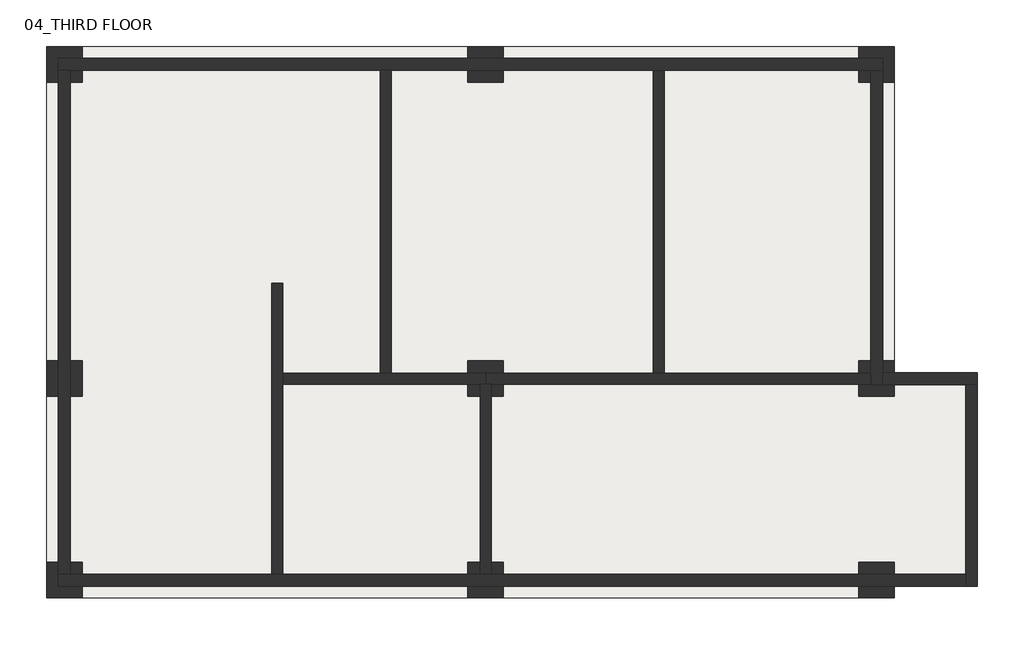
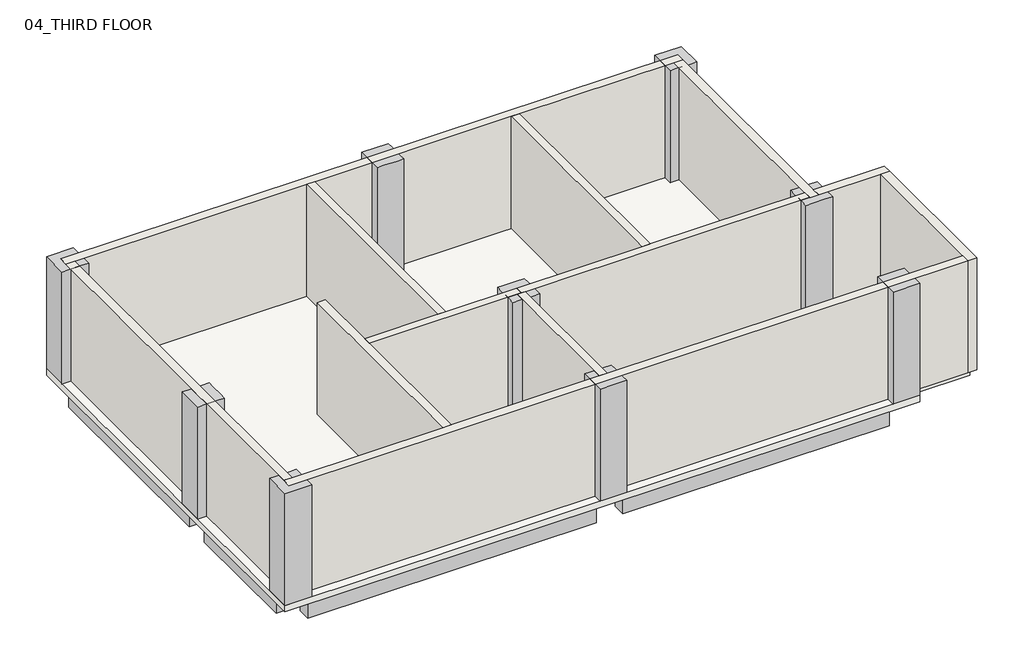
# One storey: 12 beams, 12 walls, 9 columns, 1 slab.
"""IFC4 building model written with IfcOpenShell, lengths in millimetres."""

from ifc_helpers import new_model, si_unit, frame, origin, place, context, project, spatial, polyline, outline, extrude, faceted_brep, element, save

model = new_model("IFC4")

# Units and contexts
model_context = context("Model", 3, world=origin())
ifc_project = project(units=[si_unit("LENGTHUNIT", "METRE", prefix="MILLI")], contexts=[model_context])

# Site, building, storey
site = spatial("IfcSite", under=ifc_project)
building = spatial("IfcBuilding", under=site)
storey = spatial("IfcBuildingStorey", under=building, Name="04_THIRD FLOOR", Elevation=8639.9618634)

# Beams
placement = place(None, origin())
element("IfcBeam", 1, ObjectType="RC Beam_Rectangular : H_SB_AR_S16_B300xH600", at=placement, inside=storey, context=model_context, shape_type="SweptSolid", body=[
    extrude(outline(polyline([(300.0, 1049.5208589), (300.0, 1349.5208589), (6800.0, 1349.5208589), (6800.0, 1049.5208589), (300.0, 1049.5208589)])), frame((0.0, 0.0, 8039.9618634), z_axis=(0.0, 0.0, 1.0), x_axis=(1.0, 0.0, 0.0)), (0.0, 0.0, 1.0), 450.0),
])
element("IfcBeam", 2, ObjectType="RC Beam_Rectangular : H_SB_AR_S16_B300xH600", at=placement, inside=storey, context=model_context, shape_type="SweptSolid", body=[
    extrude(outline(polyline([(7400.0, 1049.5208589), (7400.0, 1349.5208589), (13400.0, 1349.5208589), (13400.0, 1049.5208589), (7400.0, 1049.5208589)])), frame((0.0, 0.0, 8039.9618634), z_axis=(0.0, 0.0, 1.0), x_axis=(1.0, 0.0, 0.0)), (0.0, 0.0, 1.0), 450.0),
])
element("IfcBeam", 3, ObjectType="RC Beam_Rectangular : H_SB_AR_S16_B300xH600", at=placement, inside=storey, context=model_context, shape_type="SweptSolid", body=[
    extrude(outline(polyline([(300.0, 6349.5208589), (300.0, 6649.5208589), (6800.0, 6649.5208589), (6800.0, 6349.5208589), (300.0, 6349.5208589)])), frame((0.0, 0.0, 8039.9618634), z_axis=(0.0, 0.0, 1.0), x_axis=(1.0, 0.0, 0.0)), (0.0, 0.0, 1.0), 450.0),
])
element("IfcBeam", 4, ObjectType="RC Beam_Rectangular : H_SB_AR_S16_B300xH600", at=placement, inside=storey, context=model_context, shape_type="SweptSolid", body=[
    extrude(outline(polyline([(7400.0, 6349.5208589), (7400.0, 6649.5208589), (13400.0, 6649.5208589), (13400.0, 6349.5208589), (7400.0, 6349.5208589)])), frame((0.0, 0.0, 8039.9618634), z_axis=(0.0, 0.0, 1.0), x_axis=(1.0, 0.0, 0.0)), (0.0, 0.0, 1.0), 450.0),
])
element("IfcBeam", 5, ObjectType="RC Beam_Rectangular : H_SB_AR_S16_B300xH600", at=placement, inside=storey, context=model_context, shape_type="SweptSolid", body=[
    extrude(outline(polyline([(300.0, -2350.4791411), (300.0, -2050.4791411), (6800.0, -2050.4791411), (6800.0, -2350.4791411), (300.0, -2350.4791411)])), frame((0.0, 0.0, 8039.9618634), z_axis=(0.0, 0.0, 1.0), x_axis=(1.0, 0.0, 0.0)), (0.0, 0.0, 1.0), 450.0),
])
element("IfcBeam", 6, ObjectType="RC Beam_Rectangular : H_SB_AR_S16_B300xH600", at=placement, inside=storey, context=model_context, shape_type="SweptSolid", body=[
    extrude(outline(polyline([(7400.0, -2350.4791411), (7400.0, -2050.4791411), (13400.0, -2050.4791411), (13400.0, -2350.4791411), (7400.0, -2350.4791411)])), frame((0.0, 0.0, 8039.9618634), z_axis=(0.0, 0.0, 1.0), x_axis=(1.0, 0.0, 0.0)), (0.0, 0.0, 1.0), 450.0),
])
element("IfcBeam", 7, ObjectType="RC Beam_Rectangular : H_SB_AR_S16_B300xH600", at=placement, inside=storey, context=model_context, shape_type="SweptSolid", body=[
    extrude(outline(polyline([(-150.0, 899.5208589), (150.0, 899.5208589), (150.0, -1900.4791411), (-150.0, -1900.4791411), (-150.0, 899.5208589)])), frame((0.0, 0.0, 8039.9618634), z_axis=(0.0, 0.0, 1.0), x_axis=(1.0, 0.0, 0.0)), (0.0, 0.0, 1.0), 450.0),
])
element("IfcBeam", 8, ObjectType="RC Beam_Rectangular : H_SB_AR_S16_B300xH600", at=placement, inside=storey, context=model_context, shape_type="SweptSolid", body=[
    extrude(outline(polyline([(150.0, 1499.5208589), (-150.0, 1499.5208589), (-150.0, 6199.5208589), (150.0, 6199.5208589), (150.0, 1499.5208589)])), frame((0.0, 0.0, 8039.9618634), z_axis=(0.0, 0.0, 1.0), x_axis=(1.0, 0.0, 0.0)), (0.0, 0.0, 1.0), 450.0),
])
element("IfcBeam", 9, ObjectType="RC Beam_Rectangular : H_SB_AR_S16_B300xH600", at=placement, inside=storey, context=model_context, shape_type="SweptSolid", body=[
    extrude(outline(polyline([(6950.0, 899.5208589), (7250.0, 899.5208589), (7250.0, -1900.4791411), (6950.0, -1900.4791411), (6950.0, 899.5208589)])), frame((0.0, 0.0, 8039.9618634), z_axis=(0.0, 0.0, 1.0), x_axis=(1.0, 0.0, 0.0)), (0.0, 0.0, 1.0), 450.0),
])
element("IfcBeam", 10, ObjectType="RC Beam_Rectangular : H_SB_AR_S16_B300xH600", at=placement, inside=storey, context=model_context, shape_type="SweptSolid", body=[
    extrude(outline(polyline([(7250.0, 1499.5208589), (6950.0, 1499.5208589), (6950.0, 6199.5208589), (7250.0, 6199.5208589), (7250.0, 1499.5208589)])), frame((0.0, 0.0, 8039.9618634), z_axis=(0.0, 0.0, 1.0), x_axis=(1.0, 0.0, 0.0)), (0.0, 0.0, 1.0), 450.0),
])
element("IfcBeam", 11, ObjectType="RC Beam_Rectangular : H_SB_AR_S16_B300xH600", at=placement, inside=storey, context=model_context, shape_type="SweptSolid", body=[
    extrude(outline(polyline([(13550.0, 899.5208589), (13850.0, 899.5208589), (13850.0, -1900.4791411), (13550.0, -1900.4791411), (13550.0, 899.5208589)])), frame((0.0, 0.0, 8039.9618634), z_axis=(0.0, 0.0, 1.0), x_axis=(1.0, 0.0, 0.0)), (0.0, 0.0, 1.0), 450.0),
])
element("IfcBeam", 12, ObjectType="RC Beam_Rectangular : H_SB_AR_S16_B300xH600", at=placement, inside=storey, context=model_context, shape_type="SweptSolid", body=[
    extrude(outline(polyline([(13850.0, 1499.5208589), (13550.0, 1499.5208589), (13550.0, 6199.5208589), (13850.0, 6199.5208589), (13850.0, 1499.5208589)])), frame((0.0, 0.0, 8039.9618634), z_axis=(0.0, 0.0, 1.0), x_axis=(1.0, 0.0, 0.0)), (0.0, 0.0, 1.0), 450.0),
])

# Columns
element("IfcColumn", 13, ObjectType="RC_Column_Rectangular : H_SC_AR_S15_W600xL600", at=placement, inside=storey, context=model_context, shape_type="Brep", body=[
    faceted_brep([(300.0, 1499.5208589, 8639.9618634), (300.0, 899.5208589, 8639.9618634), (-300.0, 899.5208589, 8639.9618634), (-300.0, 1499.5208589, 8639.9618634), (300.0, 1499.5208589, 11309.9618634), (300.0, 1349.5208589, 11309.9618634), (300.0, 1049.5208589, 11309.9618634), (300.0, 899.5208589, 11309.9618634), (150.0, 899.5208589, 11309.9618634), (-150.0, 899.5208589, 11309.9618634), (-300.0, 899.5208589, 11309.9618634), (-300.0, 1499.5208589, 11309.9618634), (-150.0, 1499.5208589, 11309.9618634), (150.0, 1499.5208589, 11309.9618634)], [[[0, 1, 2, 3]], [[4, 5, 6, 7, 1, 0]], [[7, 8, 9, 10, 2, 1]], [[10, 11, 3, 2]], [[11, 12, 13, 4, 0, 3]], [[4, 13, 12, 11, 10, 9, 8, 7, 6, 5]]]),
])
element("IfcColumn", 14, ObjectType="RC_Column_Rectangular : H_SC_AR_S15_W600xL600", at=placement, inside=storey, context=model_context, shape_type="Brep", body=[
    faceted_brep([(7400.0, 1499.5208589, 8639.9618634), (7400.0, 899.5208589, 8639.9618634), (6800.0, 899.5208589, 8639.9618634), (6800.0, 1499.5208589, 8639.9618634), (7400.0, 1499.5208589, 11309.9618634), (7400.0, 1349.5208589, 11309.9618634), (7400.0, 1049.5208589, 11309.9618634), (7400.0, 899.5208589, 11309.9618634), (7250.0, 899.5208589, 11309.9618634), (6950.0, 899.5208589, 11309.9618634), (6800.0, 899.5208589, 11309.9618634), (6800.0, 1049.5208589, 11309.9618634), (6800.0, 1349.5208589, 11309.9618634), (6800.0, 1499.5208589, 11309.9618634), (6950.0, 1499.5208589, 11309.9618634), (7250.0, 1499.5208589, 11309.9618634)], [[[0, 1, 2, 3]], [[4, 5, 6, 7, 1, 0]], [[7, 8, 9, 10, 2, 1]], [[10, 11, 12, 13, 3, 2]], [[13, 14, 15, 4, 0, 3]], [[4, 15, 14, 13, 12, 11, 10, 9, 8, 7, 6, 5]]]),
])
element("IfcColumn", 15, ObjectType="RC_Column_Rectangular : H_SC_AR_S15_W600xL600", at=placement, inside=storey, context=model_context, shape_type="Brep", body=[
    faceted_brep([(14000.0, 1499.5208589, 8639.9618634), (14000.0, 899.5208589, 8639.9618634), (13400.0, 899.5208589, 8639.9618634), (13400.0, 1499.5208589, 8639.9618634), (14000.0, 1499.5208589, 11309.9618634), (14000.0, 1199.5208589, 11309.9618634), (14000.0, 899.5208589, 11309.9618634), (13850.0, 899.5208589, 11309.9618634), (13550.0, 899.5208589, 11309.9618634), (13400.0, 899.5208589, 11309.9618634), (13400.0, 1049.5208589, 11309.9618634), (13400.0, 1349.5208589, 11309.9618634), (13400.0, 1499.5208589, 11309.9618634), (13550.0, 1499.5208589, 11309.9618634), (13850.0, 1499.5208589, 11309.9618634)], [[[0, 1, 2, 3]], [[4, 5, 6, 1, 0]], [[6, 7, 8, 9, 2, 1]], [[9, 10, 11, 12, 3, 2]], [[12, 13, 14, 4, 0, 3]], [[4, 14, 13, 12, 11, 10, 9, 8, 7, 6, 5]]]),
])
element("IfcColumn", 16, ObjectType="RC_Column_Rectangular : H_SC_AR_S15_W600xL600", at=placement, inside=storey, context=model_context, shape_type="Brep", body=[
    faceted_brep([(300.0, 6799.5208589, 8639.9618634), (300.0, 6199.5208589, 8639.9618634), (-300.0, 6199.5208589, 8639.9618634), (-300.0, 6799.5208589, 8639.9618634), (300.0, 6799.5208589, 11309.9618634), (300.0, 6649.5208589, 11309.9618634), (300.0, 6349.5208589, 11309.9618634), (300.0, 6199.5208589, 11309.9618634), (150.0, 6199.5208589, 11309.9618634), (-150.0, 6199.5208589, 11309.9618634), (-300.0, 6199.5208589, 11309.9618634), (-300.0, 6799.5208589, 11309.9618634)], [[[0, 1, 2, 3]], [[4, 5, 6, 7, 1, 0]], [[7, 8, 9, 10, 2, 1]], [[10, 11, 3, 2]], [[11, 4, 0, 3]], [[4, 11, 10, 9, 8, 7, 6, 5]]]),
])
element("IfcColumn", 17, ObjectType="RC_Column_Rectangular : H_SC_AR_S15_W600xL600", at=placement, inside=storey, context=model_context, shape_type="Brep", body=[
    faceted_brep([(7400.0, 6799.5208589, 8639.9618634), (7400.0, 6199.5208589, 8639.9618634), (6800.0, 6199.5208589, 8639.9618634), (6800.0, 6799.5208589, 8639.9618634), (7400.0, 6799.5208589, 11309.9618634), (7400.0, 6649.5208589, 11309.9618634), (7400.0, 6349.5208589, 11309.9618634), (7400.0, 6199.5208589, 11309.9618634), (7250.0, 6199.5208589, 11309.9618634), (6950.0, 6199.5208589, 11309.9618634), (6800.0, 6199.5208589, 11309.9618634), (6800.0, 6349.5208589, 11309.9618634), (6800.0, 6649.5208589, 11309.9618634), (6800.0, 6799.5208589, 11309.9618634)], [[[0, 1, 2, 3]], [[4, 5, 6, 7, 1, 0]], [[7, 8, 9, 10, 2, 1]], [[10, 11, 12, 13, 3, 2]], [[13, 4, 0, 3]], [[4, 13, 12, 11, 10, 9, 8, 7, 6, 5]]]),
])
element("IfcColumn", 18, ObjectType="RC_Column_Rectangular : H_SC_AR_S15_W600xL600", at=placement, inside=storey, context=model_context, shape_type="Brep", body=[
    faceted_brep([(14000.0, 6799.5208589, 8639.9618634), (14000.0, 6199.5208589, 8639.9618634), (13400.0, 6199.5208589, 8639.9618634), (13400.0, 6799.5208589, 8639.9618634), (14000.0, 6799.5208589, 11309.9618634), (14000.0, 6199.5208589, 11309.9618634), (13850.0, 6199.5208589, 11309.9618634), (13550.0, 6199.5208589, 11309.9618634), (13400.0, 6199.5208589, 11309.9618634), (13400.0, 6349.5208589, 11309.9618634), (13400.0, 6649.5208589, 11309.9618634), (13400.0, 6799.5208589, 11309.9618634)], [[[0, 1, 2, 3]], [[4, 5, 1, 0]], [[5, 6, 7, 8, 2, 1]], [[8, 9, 10, 11, 3, 2]], [[11, 4, 0, 3]], [[4, 11, 10, 9, 8, 7, 6, 5]]]),
])
element("IfcColumn", 19, ObjectType="RC_Column_Rectangular : H_SC_AR_S15_W600xL600", at=placement, inside=storey, context=model_context, shape_type="Brep", body=[
    faceted_brep([(300.0, -1900.4791411, 8639.9618634), (300.0, -2500.4791411, 8639.9618634), (-300.0, -2500.4791411, 8639.9618634), (-300.0, -1900.4791411, 8639.9618634), (300.0, -1900.4791411, 11309.9618634), (300.0, -2050.4791411, 11309.9618634), (300.0, -2350.4791411, 11309.9618634), (300.0, -2500.4791411, 11309.9618634), (-300.0, -2500.4791411, 11309.9618634), (-300.0, -1900.4791411, 11309.9618634), (-150.0, -1900.4791411, 11309.9618634), (150.0, -1900.4791411, 11309.9618634)], [[[0, 1, 2, 3]], [[4, 5, 6, 7, 1, 0]], [[7, 8, 2, 1]], [[8, 9, 3, 2]], [[9, 10, 11, 4, 0, 3]], [[4, 11, 10, 9, 8, 7, 6, 5]]]),
])
element("IfcColumn", 20, ObjectType="RC_Column_Rectangular : H_SC_AR_S15_W600xL600", at=placement, inside=storey, context=model_context, shape_type="Brep", body=[
    faceted_brep([(7400.0, -1900.4791411, 8639.9618634), (7400.0, -2500.4791411, 8639.9618634), (6800.0, -2500.4791411, 8639.9618634), (6800.0, -1900.4791411, 8639.9618634), (7400.0, -1900.4791411, 11309.9618634), (7400.0, -2050.4791411, 11309.9618634), (7400.0, -2350.4791411, 11309.9618634), (7400.0, -2500.4791411, 11309.9618634), (7100.0, -2500.4791411, 11309.9618634), (6800.0, -2500.4791411, 11309.9618634), (6800.0, -2350.4791411, 11309.9618634), (6800.0, -2050.4791411, 11309.9618634), (6800.0, -1900.4791411, 11309.9618634), (6950.0, -1900.4791411, 11309.9618634), (7250.0, -1900.4791411, 11309.9618634)], [[[0, 1, 2, 3]], [[4, 5, 6, 7, 1, 0]], [[7, 8, 9, 2, 1]], [[9, 10, 11, 12, 3, 2]], [[12, 13, 14, 4, 0, 3]], [[4, 14, 13, 12, 11, 10, 9, 8, 7, 6, 5]]]),
])
element("IfcColumn", 21, ObjectType="RC_Column_Rectangular : H_SC_AR_S15_W600xL600", at=placement, inside=storey, context=model_context, shape_type="Brep", body=[
    faceted_brep([(14000.0, -1900.4791411, 8639.9618634), (14000.0, -2500.4791411, 8639.9618634), (13400.0, -2500.4791411, 8639.9618634), (13400.0, -1900.4791411, 8639.9618634), (14000.0, -1900.4791411, 11309.9618634), (14000.0, -2500.4791411, 11309.9618634), (13400.0, -2500.4791411, 11309.9618634), (13400.0, -2350.4791411, 11309.9618634), (13400.0, -2050.4791411, 11309.9618634), (13400.0, -1900.4791411, 11309.9618634), (13550.0, -1900.4791411, 11309.9618634), (13850.0, -1900.4791411, 11309.9618634)], [[[0, 1, 2, 3]], [[4, 5, 1, 0]], [[5, 6, 2, 1]], [[6, 7, 8, 9, 3, 2]], [[9, 10, 11, 4, 0, 3]], [[4, 11, 10, 9, 8, 7, 6, 5]]]),
])

# Slab
element("IfcSlab", 22, ObjectType="H_FL_AR_S17_RC Slab T150", at=placement, inside=storey, context=model_context, shape_type="SweptSolid", body=[
    extrude(outline(polyline([(14000.0, 1199.5208589), (15300.0, 1199.5208589), (15300.0, -2200.4791411), (14000.0, -2200.4791411), (14000.0, -2500.4791411), (-300.0, -2500.4791411), (-300.0, 6799.5208589), (14000.0, 6799.5208589), (14000.0, 1199.5208589)])), frame((0.0, 0.0, 8489.9618634), z_axis=(0.0, 0.0, 1.0), x_axis=(1.0, 0.0, 0.0)), (0.0, 0.0, 1.0), 150.0),
])

# Walls
element("IfcWall", 23, ObjectType="H_WA_AR_B02_Ext Wall_RC T200", at=placement, inside=storey, context=model_context, shape_type="Brep", body=[
    faceted_brep([(-100.0, 6399.5208589, 8639.9618634), (100.0, 6399.5208589, 8639.9618634), (5325.5, 6399.5208589, 8639.9618634), (5509.5, 6399.5208589, 8639.9618634), (9935.0, 6399.5208589, 8639.9618634), (10119.0, 6399.5208589, 8639.9618634), (13600.0, 6399.5208589, 8639.9618634), (13800.0, 6399.5208589, 8639.9618634), (13800.0, 6399.5208589, 11309.9618634), (13600.0, 6399.5208589, 11309.9618634), (10119.0, 6399.5208589, 11309.9618634), (9935.0, 6399.5208589, 11309.9618634), (5509.5, 6399.5208589, 11309.9618634), (5325.5, 6399.5208589, 11309.9618634), (100.0, 6399.5208589, 11309.9618634), (-100.0, 6399.5208589, 11309.9618634), (-100.0, 6599.5208589, 8639.9618634), (-100.0, 6599.5208589, 11309.9618634), (13800.0, 6599.5208589, 11309.9618634), (13800.0, 6599.5208589, 8639.9618634)], [[[0, 1, 2, 3, 4, 5, 6, 7, 8, 9, 10, 11, 12, 13, 14, 15]], [[16, 17, 18, 19]], [[7, 6, 5, 4, 3, 2, 1, 0, 16, 19]], [[15, 14, 13, 12, 11, 10, 9, 8, 18, 17]], [[8, 7, 19, 18]], [[0, 15, 17, 16]]]),
])
element("IfcWall", 24, ObjectType="H_WA_AR_B02_Ext Wall_RC T200", at=placement, inside=storey, context=model_context, shape_type="Brep", body=[
    faceted_brep([(13600.0, 6399.5208589, 8639.9618634), (13600.0, 1286.5208589, 8639.9618634), (13600.0, 1102.5208589, 8639.9618634), (13600.0, 1099.5208589, 8639.9618634), (13600.0, 1099.5208589, 11309.9618634), (13600.0, 1102.5208589, 11309.9618634), (13600.0, 1286.5208589, 11309.9618634), (13600.0, 6399.5208589, 11309.9618634), (13800.0, 6399.5208589, 8639.9618634), (13800.0, 6399.5208589, 11309.9618634), (13800.0, 1299.5208589, 11309.9618634), (13800.0, 1099.5208589, 11309.9618634), (13800.0, 1099.5208589, 8639.9618634), (13800.0, 1299.5208589, 8639.9618634)], [[[0, 1, 2, 3, 4, 5, 6, 7]], [[8, 9, 10, 11, 12, 13]], [[3, 2, 1, 0, 8, 13, 12]], [[7, 6, 5, 4, 11, 10, 9]], [[0, 7, 9, 8]], [[4, 3, 12, 11]]]),
])
element("IfcWall", 25, ObjectType="H_WA_AR_B02_Ext Wall_RC T200", at=placement, inside=storey, context=model_context, shape_type="Brep", body=[
    faceted_brep([(13800.0, 1099.5208589, 8639.9618634), (15200.0, 1099.5208589, 8639.9618634), (15400.0, 1099.5208589, 8639.9618634), (15400.0, 1099.5208589, 11309.9618634), (15200.0, 1099.5208589, 11309.9618634), (13800.0, 1099.5208589, 11309.9618634), (13800.0, 1299.5208589, 8639.9618634), (13800.0, 1299.5208589, 11309.9618634), (15400.0, 1299.5208589, 11309.9618634), (15400.0, 1299.5208589, 8639.9618634)], [[[0, 1, 2, 3, 4, 5]], [[6, 7, 8, 9]], [[2, 1, 0, 6, 9]], [[5, 4, 3, 8, 7]], [[0, 5, 7, 6]], [[3, 2, 9, 8]]]),
])
element("IfcWall", 26, ObjectType="H_WA_AR_B02_Ext Wall_RC T200", at=placement, inside=storey, context=model_context, shape_type="Brep", body=[
    faceted_brep([(15200.0, 1099.5208589, 8639.9618634), (15200.0, -2100.4791411, 8639.9618634), (15200.0, -2300.4791411, 8639.9618634), (15200.0, -2300.4791411, 11309.9618634), (15200.0, -2100.4791411, 11309.9618634), (15200.0, 1099.5208589, 11309.9618634), (15400.0, 1099.5208589, 8639.9618634), (15400.0, 1099.5208589, 11309.9618634), (15400.0, -2300.4791411, 11309.9618634), (15400.0, -2300.4791411, 8639.9618634)], [[[0, 1, 2, 3, 4, 5]], [[6, 7, 8, 9]], [[2, 1, 0, 6, 9]], [[5, 4, 3, 8, 7]], [[0, 5, 7, 6]], [[3, 2, 9, 8]]]),
])
element("IfcWall", 27, ObjectType="H_WA_AR_B02_Ext Wall_RC T200", at=placement, inside=storey, context=model_context, shape_type="Brep", body=[
    faceted_brep([(15200.0, -2100.4791411, 8639.9618634), (7197.0, -2100.4791411, 8639.9618634), (7013.0, -2100.4791411, 8639.9618634), (3680.0, -2100.4791411, 8639.9618634), (3496.0, -2100.4791411, 8639.9618634), (100.0, -2100.4791411, 8639.9618634), (-100.0, -2100.4791411, 8639.9618634), (-100.0, -2100.4791411, 11309.9618634), (100.0, -2100.4791411, 11309.9618634), (3496.0, -2100.4791411, 11309.9618634), (3680.0, -2100.4791411, 11309.9618634), (7013.0, -2100.4791411, 11309.9618634), (7197.0, -2100.4791411, 11309.9618634), (15200.0, -2100.4791411, 11309.9618634), (15200.0, -2300.4791411, 8639.9618634), (15200.0, -2300.4791411, 11309.9618634), (-100.0, -2300.4791411, 11309.9618634), (-100.0, -2300.4791411, 8639.9618634)], [[[0, 1, 2, 3, 4, 5, 6, 7, 8, 9, 10, 11, 12, 13]], [[14, 15, 16, 17]], [[6, 5, 4, 3, 2, 1, 0, 14, 17]], [[13, 12, 11, 10, 9, 8, 7, 16, 15]], [[0, 13, 15, 14]], [[7, 6, 17, 16]]]),
])
element("IfcWall", 28, ObjectType="H_WA_AR_B02_Ext Wall_RC T200", at=placement, inside=storey, context=model_context, shape_type="SweptSolid", body=[
    extrude(outline(polyline([(100.0, 6399.5208589), (100.0, -2100.4791411), (-100.0, -2100.4791411), (-100.0, 6399.5208589), (100.0, 6399.5208589)])), frame((0.0, 0.0, 8639.9618634), z_axis=(0.0, 0.0, 1.0), x_axis=(1.0, 0.0, 0.0)), (0.0, 0.0, 1.0), 2670.0),
])
element("IfcWall", 29, ObjectType="H_WA_AR_B02_Int Wall_Block T150", at=placement, inside=storey, context=model_context, shape_type="Brep", body=[
    faceted_brep([(7197.0, -2100.4791411, 8639.9618634), (7197.0, 1102.5208589, 8639.9618634), (7197.0, 1102.5208589, 11309.9618634), (7197.0, -2100.4791411, 11309.9618634), (7013.0, -2100.4791411, 8639.9618634), (7013.0, -2100.4791411, 11309.9618634), (7013.0, 1102.5208589, 11309.9618634), (7013.0, 1102.5208589, 8639.9618634), (7105.0, 1102.5208589, 8639.9618634), (7105.0, 1102.5208589, 11309.9618634)], [[[0, 1, 2, 3]], [[4, 5, 6, 7]], [[1, 0, 4, 7, 8]], [[3, 2, 9, 6, 5]], [[0, 3, 5, 4]], [[2, 1, 8, 7, 6, 9]]]),
])
element("IfcWall", 30, ObjectType="H_WA_AR_B02_Int Wall_Block T150", at=placement, inside=storey, context=model_context, shape_type="Brep", body=[
    faceted_brep([(7105.0, 1102.5208589, 8639.9618634), (7197.0, 1102.5208589, 8639.9618634), (13600.0, 1102.5208589, 8639.9618634), (13600.0, 1102.5208589, 11309.9618634), (7197.0, 1102.5208589, 11309.9618634), (7105.0, 1102.5208589, 11309.9618634), (7105.0, 1286.5208589, 8639.9618634), (7105.0, 1286.5208589, 11309.9618634), (9935.0, 1286.5208589, 11309.9618634), (10119.0, 1286.5208589, 11309.9618634), (13600.0, 1286.5208589, 11309.9618634), (13600.0, 1286.5208589, 8639.9618634), (10119.0, 1286.5208589, 8639.9618634), (9935.0, 1286.5208589, 8639.9618634)], [[[0, 1, 2, 3, 4, 5]], [[6, 7, 8, 9, 10, 11, 12, 13]], [[2, 1, 0, 6, 13, 12, 11]], [[5, 4, 3, 10, 9, 8, 7]], [[0, 5, 7, 6]], [[3, 2, 11, 10]]]),
])
element("IfcWall", 31, ObjectType="H_WA_AR_B02_Int Wall_Block T150", at=placement, inside=storey, context=model_context, shape_type="Brep", body=[
    faceted_brep([(3496.0, 2811.5208589, 8639.9618634), (3496.0, -2100.4791411, 8639.9618634), (3496.0, -2100.4791411, 11309.9618634), (3496.0, 2811.5208589, 11309.9618634), (3680.0, 2811.5208589, 8639.9618634), (3680.0, 2811.5208589, 11309.9618634), (3680.0, 1286.5208589, 11309.9618634), (3680.0, 1102.5208589, 11309.9618634), (3680.0, -2100.4791411, 11309.9618634), (3680.0, -2100.4791411, 8639.9618634), (3680.0, 1102.5208589, 8639.9618634), (3680.0, 1286.5208589, 8639.9618634)], [[[0, 1, 2, 3]], [[4, 5, 6, 7, 8, 9, 10, 11]], [[1, 0, 4, 11, 10, 9]], [[3, 2, 8, 7, 6, 5]], [[0, 3, 5, 4]], [[2, 1, 9, 8]]]),
])
element("IfcWall", 32, ObjectType="H_WA_AR_B02_Int Wall_Block T150", at=placement, inside=storey, context=model_context, shape_type="Brep", body=[
    faceted_brep([(3680.0, 1102.5208589, 8639.9618634), (7105.0, 1102.5208589, 8639.9618634), (7105.0, 1102.5208589, 11309.9618634), (3680.0, 1102.5208589, 11309.9618634), (3680.0, 1286.5208589, 8639.9618634), (3680.0, 1286.5208589, 11309.9618634), (5325.5, 1286.5208589, 11309.9618634), (5509.5, 1286.5208589, 11309.9618634), (7105.0, 1286.5208589, 11309.9618634), (7105.0, 1286.5208589, 8639.9618634), (5509.5, 1286.5208589, 8639.9618634), (5325.5, 1286.5208589, 8639.9618634)], [[[0, 1, 2, 3]], [[4, 5, 6, 7, 8, 9, 10, 11]], [[1, 0, 4, 11, 10, 9]], [[2, 1, 9, 8]], [[3, 2, 8, 7, 6, 5]], [[0, 3, 5, 4]]]),
])
element("IfcWall", 33, ObjectType="H_WA_AR_B02_Int Wall_Block T150", at=placement, inside=storey, context=model_context, shape_type="SweptSolid", body=[
    extrude(outline(polyline([(5509.5, 6399.5208589), (5509.5, 1286.5208589), (5325.5, 1286.5208589), (5325.5, 6399.5208589), (5509.5, 6399.5208589)])), frame((0.0, 0.0, 8639.9618634), z_axis=(0.0, 0.0, 1.0), x_axis=(1.0, 0.0, 0.0)), (0.0, 0.0, 1.0), 2670.0),
])
element("IfcWall", 34, ObjectType="H_WA_AR_B02_Int Wall_Block T150", at=placement, inside=storey, context=model_context, shape_type="SweptSolid", body=[
    extrude(outline(polyline([(10119.0, 6399.5208589), (10119.0, 1286.5208589), (9935.0, 1286.5208589), (9935.0, 6399.5208589), (10119.0, 6399.5208589)])), frame((0.0, 0.0, 8639.9618634), z_axis=(0.0, 0.0, 1.0), x_axis=(1.0, 0.0, 0.0)), (0.0, 0.0, 1.0), 2670.0),
])

save(model, "model.ifc")

# Revit data of these elements
# Type "RC Beam_Rectangular : H_SB_AR_S16_B300xH600"
#   중앙부 하부근 = ""
#   중앙부 상부근 = ""
#   중앙부 보조근 = ""
#   중앙부 늑근 = ""
#   외단부 하부근 = ""
#   외단부 상부근 = ""
#   외단부 보조근 = ""
#   외단부 늑근 = ""
#   부호 = "TG3"
#   내단부 하부근 = ""
#   내단부 상부근 = ""
#   내단부 보조근 = ""
#   내단부 늑근 = ""
#   ALL 하부근 = "3-D20"
#   ALL 상부근 = "3-D20"
#   ALL 보조근 = ""
#   ALL 늑근 = "2-D10 @120"
#   Width = 300 mm
#   Height = 600 mm
#   Length [instance default] = 1524 mm
#   b = 300 mm
#   h = 600 mm
#   hec_material3 [instance default] = none
#   hec_material2 [instance default] = none
#   hec_material1 [instance default] = none
#   Structural Material [instance default] = none
#   Assembly Code = ""
# Type "RC_Column_Rectangular : H_SC_AR_S15_W600xL600"
#   Width = 600 mm
#   Length = 600 mm
#   hec_material3 [instance default] = none
#   hec_material2 [instance default] = none
#   hec_material1 [instance default] = none
#   Structural Material [instance default] = none
#   Description = (empty or 0)
# Type "H_FL_AR_S17_RC Slab T150"
#   Keynote = ""
#   Type Comments = ""
#   Description = ""
#   Function = 1
#   Layers, outside or top first: 150 mm no material (function 1)
# Type "H_WA_AR_B02_Ext Wall_RC T200"
#   Type Comments = ""
#   Layers, outside or top first: 0 mm no material (function 100); 0 mm no material (function 100); 200 mm no material (function 1); 0 mm no material (function 100); 0 mm no material (function 100); 0 mm no material (function 100)
# Type "H_WA_AR_B02_Int Wall_Block T150"
#   Type Comments = ""
#   Layers, outside or top first: 0 mm no material (function 100); 12 mm no material (function 2); 150 mm no material (function 1); 12 mm no material (function 2); 10 mm no material (function 5)
# Elements 1, 2, 3, 4, 5, 6, 7, 8, 9, 10, 11, 12 (IfcBeam, "RC Beam_Rectangular : H_SB_AR_S16_B300xH600")
#   Comments = ""
#   hec_material3 = none
#   hec_material2 = none
#   hec_material1 = none
#   Structural Material = none
#   Phase Created = New Construction
# Elements 13, 14, 15, 16, 17, 18, 19, 20, 21 (IfcColumn, "RC_Column_Rectangular : H_SC_AR_S15_W600xL600")
#   Comments = ""
#   hec_material3 = none
#   hec_material2 = none
#   hec_material1 = none
#   Structural Material = none
#   Phase Created = New Construction
# Element 22 (IfcSlab, "H_FL_AR_S17_RC Slab T150")
#   Height Offset From Level = 0 mm
#   Phase Created = New Construction
#   Materials on its faces: "Default Floor"
# Elements 23, 24, 25, 26, 27, 28 (IfcWall, "H_WA_AR_B02_Ext Wall_RC T200")
#   Top Offset = 0 mm
#   Base Offset = 0 mm
#   wall height = 2670 mm
#   Phase Created = New Construction
#   Base Constraint = 04_THIRD FLOOR
#   Top Constraint = 05_FOURTH FLOOR/TOP OF ROOF
#   Materials on its faces: "Default Wall"
# Elements 29, 30, 31, 32, 33, 34 (IfcWall, "H_WA_AR_B02_Int Wall_Block T150")
#   Top Offset = 0 mm
#   Base Offset = 0 mm
#   wall height = 2670 mm
#   Phase Created = New Construction
#   Base Constraint = 04_THIRD FLOOR
#   Top Constraint = 05_FOURTH FLOOR/TOP OF ROOF
#   Materials on its faces: "Default Wall"
# Materials
#   "Default Floor": class "Miscellaneous", colour RGB 80 80 80, transparency 0
#   "Default Wall": class "Miscellaneous", colour RGB 80 80 80, transparency 0
# Room at (11202.5, -500.479) mm, phase "New Construction", upper level "05_FOURTH FLOOR/TOP OF ROOF", upper offset 1000 mm, lower offset -1000 mm
#   Comments = ""
#   Number = "140"
#   Name = "STAIRS"
# Room at (5346.5, -502.979) mm, phase "New Construction", upper level "05_FOURTH FLOOR/TOP OF ROOF", upper offset 1000 mm, lower offset -1000 mm
#   Comments = ""
#   Number = "141"
#   Name = "TECHNICAL TOWER"
# Room at (2708.75, 2149.521) mm, phase "New Construction", upper level "05_FOURTH FLOOR/TOP OF ROOF", upper offset 1000 mm, lower offset -1000 mm
#   Comments = ""
#   Number = "142"
#   Name = "CARBONACEOUS FIRE ROOM"
# Room at (7722.25, 3847.021) mm, phase "New Construction", upper level "05_FOURTH FLOOR/TOP OF ROOF", upper offset 1000 mm, lower offset -1000 mm
#   Comments = ""
#   Number = "143"
#   Name = "LPG FIRE ROOM"
# Room at (11863.5, 3847.021) mm, phase "New Construction", upper level "05_FOURTH FLOOR/TOP OF ROOF", upper offset 1000 mm, lower offset -1000 mm
#   Comments = ""
#   Number = "144"
#   Name = "LOBBY"
